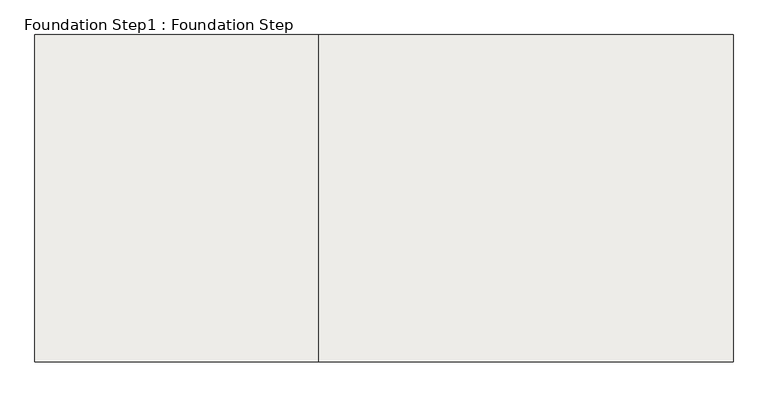
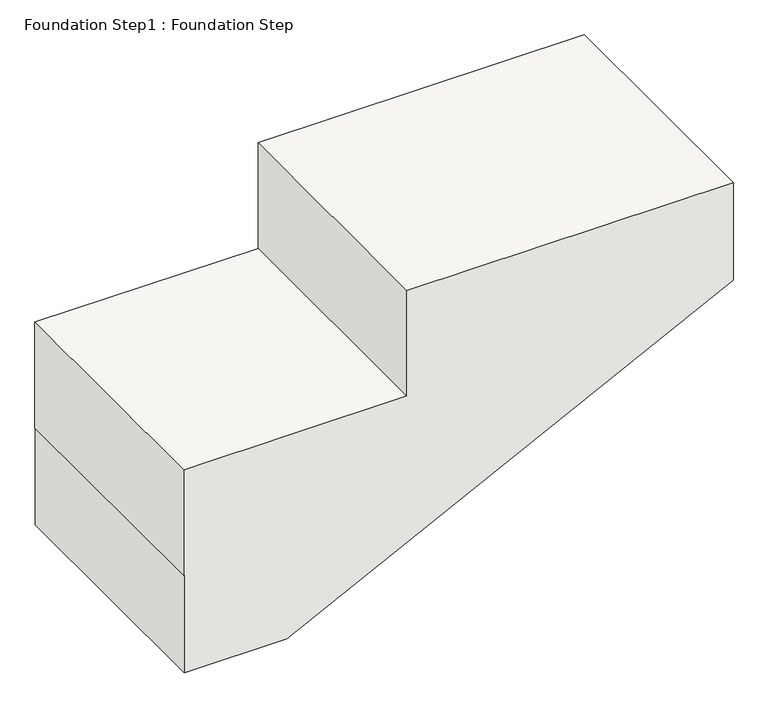
"""IFC4 building model written with IfcOpenShell, lengths in millimetres: slab geometry, Foundation Step1 : Foundation Step."""

from ifc_helpers import new_model, si_unit, frame, origin, place, context, project, spatial, polyline, outline, extrude, source, transform, mapped, element, save


def foundation_step1_foundation_step_c4984ecd(model_context):
    return source(origin(), model_context, "Body", "SweptSolid", [
        extrude(outline(polyline([(-1397.0, -62011.044558), (-1092.2, -62011.044558), (-1092.2, -62976.244558), (-1422.4, -62976.244558), (-1422.4, -63636.644558), (-1752.6, -63636.644558), (-1752.6, -63634.9850821), (-2057.4, -63634.9850821), (-2057.4, -63331.844558), (-1397.0, -62011.044558)])), frame((0.0, 12612.4268471, 0.0), z_axis=(0.0, 1.0, 0.0), x_axis=(0.0, 0.0, 1.0)), (0.0, 0.0, 1.0), 762.0),
    ])


if __name__ == "__main__":
    model = new_model("IFC4")
    model_context = context("Model", 3, world=origin())
    ifc_project = project(units=[si_unit("LENGTHUNIT", "METRE", prefix="MILLI")], contexts=[model_context])
    site = spatial("IfcSite", under=ifc_project)
    building = spatial("IfcBuilding", under=site)
    placement = place(None, origin())
    foundation_step1_foundation_step_shape = foundation_step1_foundation_step_c4984ecd(model_context)
    element("IfcSlab", 1, ObjectType="Foundation Step1 : Foundation Step", at=placement, inside=building, context=model_context, shape_type="MappedRepresentation", body=[
        mapped(foundation_step1_foundation_step_shape, transform((0.0, 0.0, 0.0), x_axis=(1.0, 0.0, 0.0), y_axis=(0.0, 1.0, 0.0), z_axis=(0.0, 0.0, 1.0))),
    ])
    save(model, "model.ifc")

# Revit data of these elements
# Type "Foundation Step1 : Foundation Step"
#   Structural Material = Concrete, Cast-in-Place gray
# Materials
#   "Concrete, Cast-in-Place gray": class "Concrete", colour RGB 192 192 192, transparency 0, Description = "Cast-in-place concrete", Cost = 0
